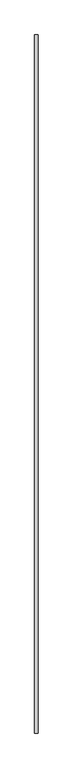
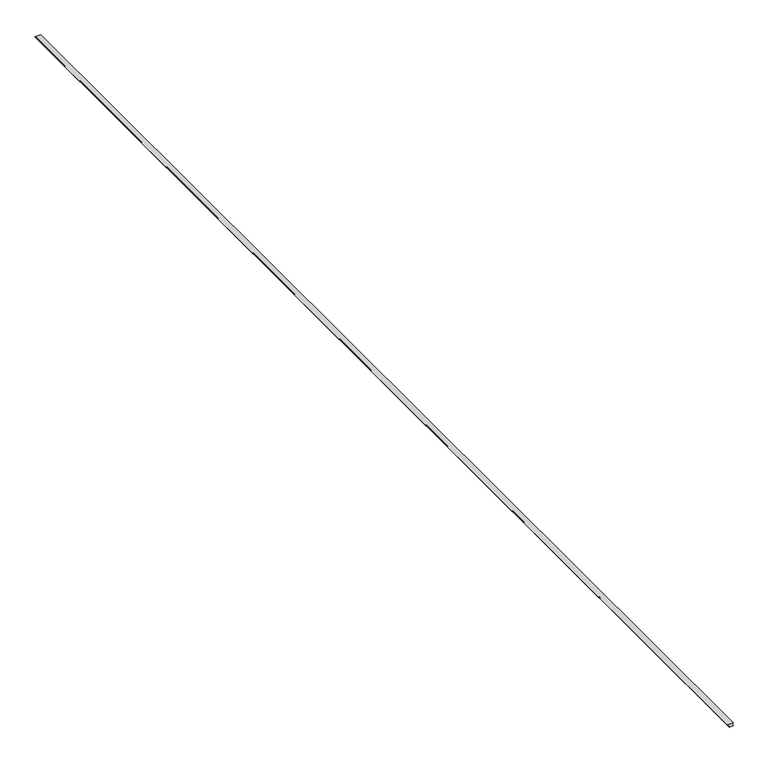
"""IFC4 building model written with IfcOpenShell, lengths in millimetres: proxy geometry, Joint024 15266 : Joint024 15266."""

from ifc_helpers import new_model, si_unit, point, frame, frame_2d, origin, place, context, project, spatial, polyline, circle_curve, trimmed, segment, composite_curve, outline, extrude, source, transform, mapped, element, save


def generic_models_f5bc10d6(model_context):
    return source(origin(), model_context, "Body", "SweptSolid", [
        extrude(outline(composite_curve([segment(polyline([(42101.9016246, -987.3744125), (42101.9016246, -997.2971191)]), True, "CONTINUOUS"), segment(trimmed(circle_curve(frame_2d((42095.7772576, -1000.721592)), 7.0167574), [point((42101.9016246, -997.2971191))], [point((42096.3078126, -993.7249216))], True, "CARTESIAN"), True, "CONTINUOUS"), segment(polyline([(42096.3078126, -993.7249216), (42096.3078142, -987.3744125)]), True, "CONTINUOUS"), segment(trimmed(circle_curve(frame_2d((42099.1047194, -983.3372169)), 4.9113773), [point((42096.3078142, -987.3744125))], [point((42101.9016246, -987.3744125))], True, "CARTESIAN"), True, "CONTINUOUS")], self_intersect=False)), frame((0.0, -1052.8906544, 0.0), z_axis=(0.0, 1.0, 0.0), x_axis=(0.0, 0.0, 1.0)), (0.0, 0.0, 1.0), 2000.0),
    ])


if __name__ == "__main__":
    model = new_model("IFC4")
    model_context = context("Model", 3, world=origin())
    ifc_project = project(units=[si_unit("LENGTHUNIT", "METRE", prefix="MILLI")], contexts=[model_context])
    site = spatial("IfcSite", under=ifc_project)
    building = spatial("IfcBuilding", under=site)
    placement = place(None, origin())
    generic_models_shape = generic_models_f5bc10d6(model_context)
    element("IfcBuildingElementProxy", 1, Name="Joint024 15266 : Joint024 15266", ObjectType="Joint024 15266 : Joint024 15266", at=placement, inside=building, context=model_context, shape_type="MappedRepresentation", body=[
        mapped(generic_models_shape, transform((0.0, 0.0, 0.0), x_axis=(1.0, 0.0, 0.0), y_axis=(0.0, 1.0, 0.0), z_axis=(0.0, 0.0, 1.0))),
    ])
    save(model, "model.ifc")

# Revit data of these elements
# Type "Joint024 15266 : Joint024 15266"
#   NameOverride = "Joint024"
# Element 1 (IfcBuildingElementProxy, "Joint024 15266 : Joint024 15266")
#   Materials on its faces: "SEALANT"
# Materials
#   "SEALANT": class "Unassigned", colour RGB 142 225 148, transparency 0
